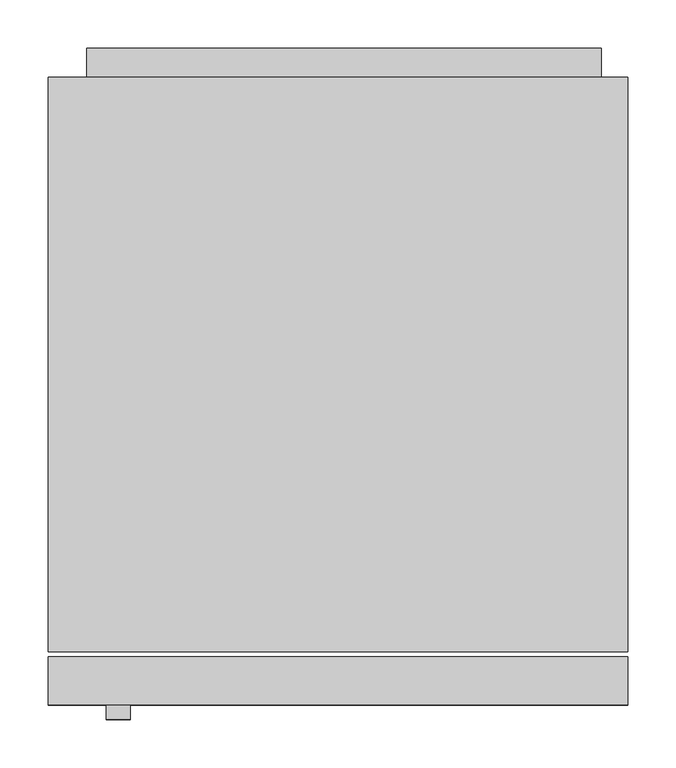
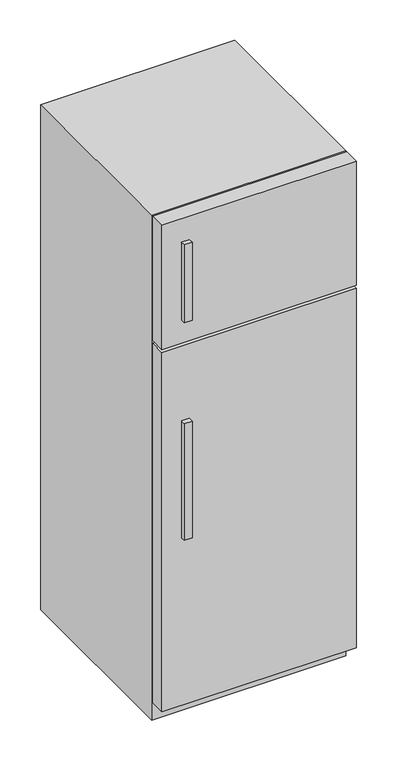
"""IFC4 building model written with IfcOpenShell, lengths in millimetres: proxy geometry, .GELADEIRA : Geladeira."""

from ifc_helpers import new_model, si_unit, frame, origin, origin_with_axes, place, context, project, spatial, polyline, outline, extrude, source, transform, mapped, element, save


def specialty_equipment_761eefd1(model_context):
    return source(origin(), model_context, "Body", "SweptSolid", [
        extrude(outline(polyline([(84.664069, 97.0), (60.0, 97.0), (60.0, 112.0), (84.664069, 112.0), (84.664069, 97.0)])), frame((0.0, 0.0, 1320.0), z_axis=(0.0, 0.0, 1.0), x_axis=(1.0, 0.0, 0.0)), (0.0, 0.0, 1.0), 254.0),
        extrude(outline(polyline([(84.664069, 97.0), (60.0, 97.0), (60.0, 112.0), (84.664069, 112.0), (84.664069, 97.0)])), frame((0.0, 0.0, 609.0), z_axis=(0.0, 0.0, 1.0), x_axis=(1.0, 0.0, 0.0)), (0.0, 0.0, 1.0), 381.0),
        extrude(outline(polyline([(600.0, 112.0), (0.0, 112.0), (0.0, 162.0), (600.0, 162.0), (600.0, 112.0)])), frame((0.0, 0.0, 1244.0), z_axis=(0.0, 0.0, 1.0), x_axis=(1.0, 0.0, 0.0)), (0.0, 0.0, 1.0), 406.0),
        extrude(outline(polyline([(600.0, 112.0), (0.0, 112.0), (0.0, 162.0), (600.0, 162.0), (600.0, 112.0)])), frame((0.0, 0.0, 60.0), z_axis=(0.0, 0.0, 1.0), x_axis=(1.0, 0.0, 0.0)), (0.0, 0.0, 1.0), 1174.0),
        extrude(outline(polyline([(600.0, 762.0), (600.0, 167.0), (0.0, 167.0), (0.0, 762.0), (600.0, 762.0)])), origin_with_axes(), (0.0, 0.0, 1.0), 1650.0),
        extrude(outline(polyline([(572.6117178, 792.0), (572.6117178, 762.0), (40.0, 762.0), (40.0, 792.0), (572.6117178, 792.0)])), frame((0.0, 0.0, 187.633046), z_axis=(0.0, 0.0, 1.0), x_axis=(1.0, 0.0, 0.0)), (0.0, 0.0, 1.0), 1132.366954),
    ])


if __name__ == "__main__":
    model = new_model("IFC4")
    model_context = context("Model", 3, world=origin())
    ifc_project = project(units=[si_unit("LENGTHUNIT", "METRE", prefix="MILLI")], contexts=[model_context])
    site = spatial("IfcSite", under=ifc_project)
    building = spatial("IfcBuilding", under=site)
    placement = place(None, origin())
    specialty_equipment_shape = specialty_equipment_761eefd1(model_context)
    element("IfcBuildingElementProxy", 1, Name=".GELADEIRA : Geladeira", ObjectType=".GELADEIRA : Geladeira", at=placement, inside=building, context=model_context, shape_type="MappedRepresentation", body=[
        mapped(specialty_equipment_shape, transform((0.0, 0.0, 0.0), x_axis=(1.0, 0.0, 0.0), y_axis=(0.0, 1.0, 0.0), z_axis=(0.0, 0.0, 1.0))),
    ])
    save(model, "model.ifc")

# Revit data of these elements
# Type ".GELADEIRA : Geladeira"
#   Marca = "Brastemp"
#   Keynote = "N"
#   Profundidade = 0.65 m
#   Altura = 1.65 m
#   Largura = 0.60 m
#   Material = Pintura geladeira
# Element 1 (IfcBuildingElementProxy, ".GELADEIRA : Geladeira")
#   Materials on its faces: "Pintura geladeira", "Metal - Chrome"
# Materials
#   "Pintura geladeira": class "Paint", colour RGB 247 247 239, transparency 0, Cost = 0
#   "Metal - Chrome": class "Unassigned", colour RGB 17 17 17, transparency 0, Description = "Chrome"
